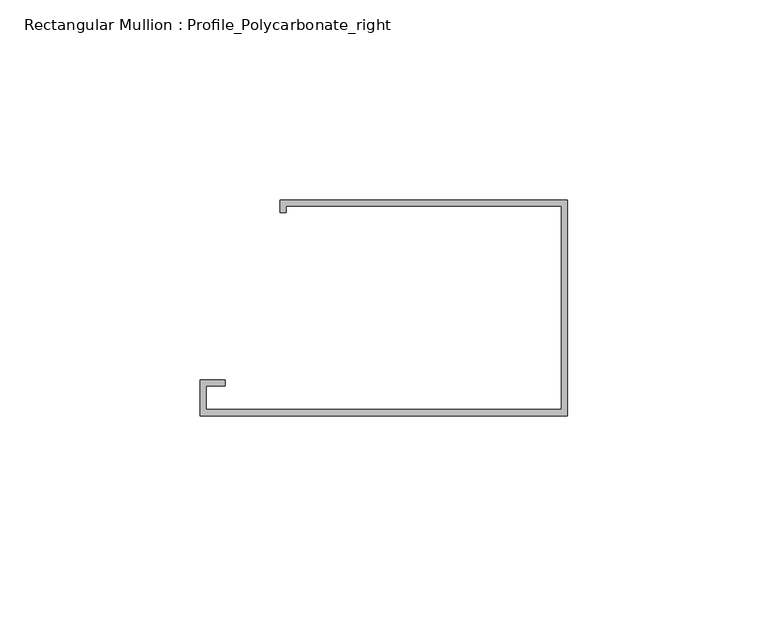
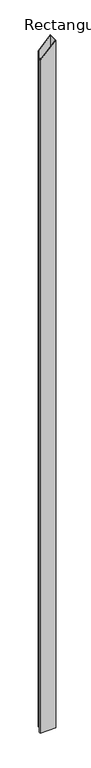
"""IFC4 building model written with IfcOpenShell, lengths in millimetres: member geometry, Rectangular Mullion : Profile_Polycarbonate_right."""

from ifc_helpers import new_model, si_unit, origin, place, context, project, spatial, faceted_brep, source, transform, mapped, element, save


def rectangular_mullion_profile_polycarbonate_right_cfd86602(model_context):
    return source(origin(), model_context, "Body", "Brep", [
        faceted_brep([(0.0, -28.984575, -4328.0127603), (-91.9988, -28.984575, -4328.0127603), (-91.9988, -19.992975, -4328.0127603), (-85.6488, -19.992975, -4328.0127603), (-85.6488, -21.580475, -4328.0127603), (-90.4113, -21.580475, -4328.0127603), (-90.4113, -27.397075, -4328.0127603), (-1.5875, -27.397075, -4328.0127603), (-1.5875, 23.428325, -4328.0127603), (-70.3961, 23.428325, -4328.0127603), (-70.3961, 21.840825, -4328.0127603), (-71.9836, 21.840825, -4328.0127603), (-71.9836, 25.015825, -4328.0127603), (0.0, 25.015825, -4328.0127603), (0.0, 25.015825, 0.0), (0.0, -28.984575, 0.0), (-71.9836, 25.015825, -75.0453753), (-71.9836, 21.840825, -75.0453753), (-70.3961, 21.840825, -73.3903521), (-70.3961, 23.428325, -73.3903521), (-1.5875, 23.428325, -1.6550233), (-1.5875, -27.397075, -1.6550233), (-90.4113, -27.397075, -94.2568855), (-90.4113, -21.580475, -94.2568855), (-85.6488, -21.580475, -89.2918157), (-85.6488, -19.992975, -89.2918157), (-91.9988, -19.992975, -95.9119088), (-91.9988, -28.984575, -95.9119088)], [[[0, 1, 2, 3, 4, 5, 6, 7, 8, 9, 10, 11, 12, 13]], [[14, 15, 0, 13]], [[16, 14, 13, 12]], [[17, 16, 12, 11]], [[18, 17, 11, 10]], [[19, 18, 10, 9]], [[20, 19, 9, 8]], [[21, 20, 8, 7]], [[22, 21, 7, 6]], [[23, 22, 6, 5]], [[24, 23, 5, 4]], [[25, 24, 4, 3]], [[26, 25, 3, 2]], [[27, 26, 2, 1]], [[15, 27, 1, 0]], [[15, 14, 16, 17, 18, 19, 20, 21, 22, 23, 24, 25, 26, 27]]]),
    ])


if __name__ == "__main__":
    model = new_model("IFC4")
    model_context = context("Model", 3, world=origin())
    ifc_project = project(units=[si_unit("LENGTHUNIT", "METRE", prefix="MILLI")], contexts=[model_context])
    site = spatial("IfcSite", under=ifc_project)
    building = spatial("IfcBuilding", under=site)
    placement = place(None, origin())
    rectangular_mullion_profile_polycarbonate_right_shape = rectangular_mullion_profile_polycarbonate_right_cfd86602(model_context)
    element("IfcMember", 1, ObjectType="Rectangular Mullion : Profile_Polycarbonate_right", at=placement, inside=building, context=model_context, shape_type="MappedRepresentation", body=[
        mapped(rectangular_mullion_profile_polycarbonate_right_shape, transform((0.0, 0.0, 0.0), x_axis=(1.0, 0.0, 0.0), y_axis=(0.0, 1.0, 0.0), z_axis=(0.0, 0.0, 1.0))),
    ])
    save(model, "model.ifc")

# Revit data of these elements
# Type "Rectangular Mullion : Profile_Polycarbonate_right"
#   built-in parameter 1007322 = 0.177167 (stored number, unit not read)
#   built-in parameter 1007321 = 0 (stored number, unit not read)
#   built-in parameter 1007320 = 0.00520833 (stored number, unit not read)
